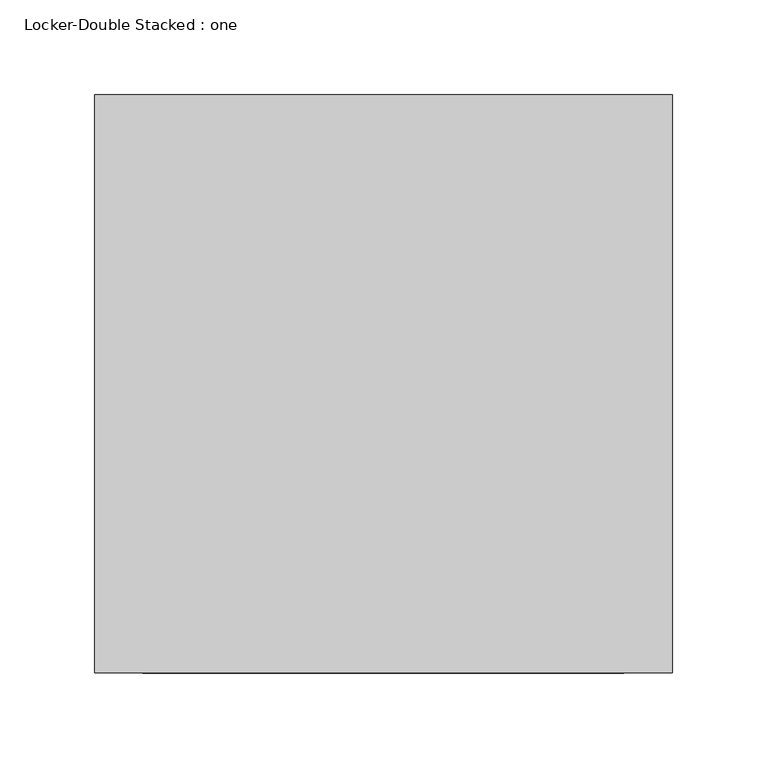
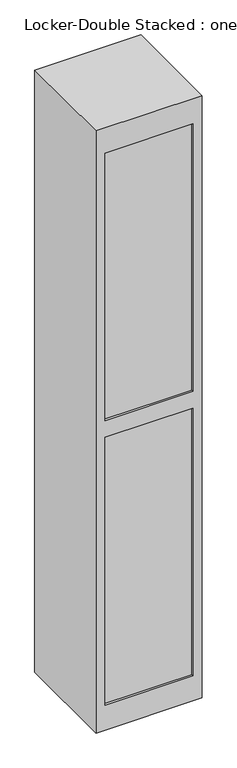
"""IFC4 building model written with IfcOpenShell, lengths in millimetres: furniture geometry, Locker-Double Stacked : one."""

from ifc_helpers import new_model, si_unit, origin, place, context, project, spatial, faceted_brep, source, transform, mapped, element, save


def locker_double_stacked_one_200c970f(model_context):
    return source(origin(), model_context, "Body", "Brep", [
        faceted_brep([(152.4, -152.4, 1828.8), (152.4, 152.4, 1828.8), (-152.4, 152.4, 1828.8), (-152.4, -152.4, 1828.8), (152.4, -152.4, 0.0), (-152.4, -152.4, 0.0), (-152.4, 152.4, 0.0), (152.4, 152.4, 0.0), (127.0, -152.4, 889.0), (127.0, -152.4, 76.2), (-127.0, -152.4, 76.2), (-127.0, -152.4, 889.0), (-127.0, -152.4, 1752.6), (127.0, -152.4, 1752.6), (127.0, -152.4, 939.8), (-127.0, -152.4, 939.8), (127.0, -146.05, 76.2), (127.0, -146.05, 889.0), (-127.0, -146.05, 889.0), (-127.0, -146.05, 76.2), (127.0, -146.05, 1752.6), (-127.0, -146.05, 1752.6), (-127.0, -146.05, 939.8), (127.0, -146.05, 939.8)], [[[0, 1, 2, 3]], [[4, 5, 6, 7]], [[1, 0, 4, 7]], [[2, 1, 7, 6]], [[3, 2, 6, 5]], [[0, 3, 5, 4], [8, 9, 10, 11], [12, 13, 14, 15]], [[16, 17, 18, 19]], [[17, 16, 9, 8]], [[18, 17, 8, 11]], [[19, 18, 11, 10]], [[16, 19, 10, 9]], [[20, 21, 22, 23]], [[21, 20, 13, 12]], [[22, 21, 12, 15]], [[23, 22, 15, 14]], [[20, 23, 14, 13]]]),
    ])


if __name__ == "__main__":
    model = new_model("IFC4")
    model_context = context("Model", 3, world=origin())
    ifc_project = project(units=[si_unit("LENGTHUNIT", "METRE", prefix="MILLI")], contexts=[model_context])
    site = spatial("IfcSite", under=ifc_project)
    building = spatial("IfcBuilding", under=site)
    placement = place(None, origin())
    locker_double_stacked_one_shape = locker_double_stacked_one_200c970f(model_context)
    element("IfcFurniture", 1, ObjectType="Locker-Double Stacked : one", at=placement, inside=building, context=model_context, shape_type="MappedRepresentation", body=[
        mapped(locker_double_stacked_one_shape, transform((0.0, 0.0, 0.0), x_axis=(1.0, 0.0, 0.0), y_axis=(0.0, 1.0, 0.0), z_axis=(0.0, 0.0, 1.0))),
    ])
    save(model, "model.ifc")

# Revit data of these elements
# Project information
#   Project Issue Date = "Issue Date"
#   Project Status = "Project Status"
#   Client Name = "Owner"
#   Project Address = "Enter address here"
#   Project Name = "6060 McKee Rd, Fitchburg, WI 53719"
#   Project Number = "Project Number"
# Type "Locker-Double Stacked : one"
#   Keynote = "M10511300.01"
#   Keynote = "M10511300.01"
#   Assembly Code = "E2010"
#   Depth = 1' - 0"
#   Height = 6' - 0"
#   Width = 1' - 0"
#   Material = LOCKERS
# Element 1 (IfcFurniture, "Locker-Double Stacked : one")
#   Materials on its faces: "LOCKERS"
# Materials
#   "LOCKERS": class "Unassigned", colour RGB 98 98 98, transparency 0, Description = "Metal Painted", Cost = 0
